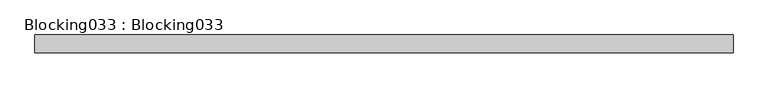
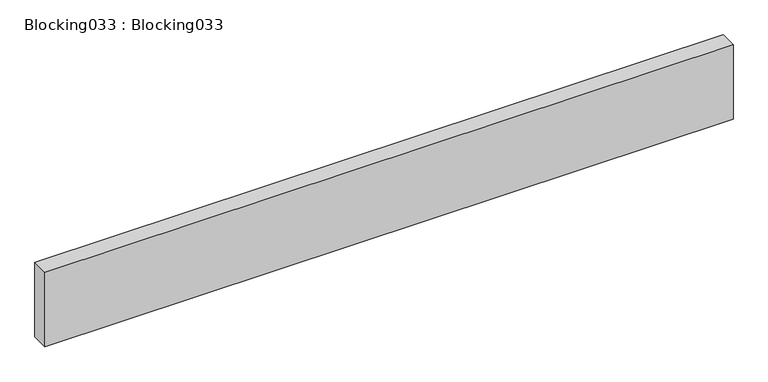
"""IFC4 building model written with IfcOpenShell, lengths in millimetres: proxy geometry, Blocking033 : Blocking033."""

from ifc_helpers import new_model, si_unit, frame, origin, place, context, project, spatial, polyline, outline, extrude, source, transform, mapped, element, save


def blocking033_blocking033_df2a4a9a(model_context):
    return source(origin(), model_context, "Body", "SweptSolid", [
        extrude(outline(polyline([(3694.2883192, 9592.4838724), (3694.2883192, 9643.2838724), (5694.2883192, 9643.2838724), (5694.2883192, 9592.4838724), (3694.2883192, 9592.4838724)])), frame((0.0, 0.0, 39528.496), z_axis=(0.0, 0.0, 1.0), x_axis=(1.0, 0.0, 0.0)), (0.0, 0.0, 1.0), 228.6),
    ])


if __name__ == "__main__":
    model = new_model("IFC4")
    model_context = context("Model", 3, world=origin())
    ifc_project = project(units=[si_unit("LENGTHUNIT", "METRE", prefix="MILLI")], contexts=[model_context])
    site = spatial("IfcSite", under=ifc_project)
    building = spatial("IfcBuilding", under=site)
    placement = place(None, origin())
    blocking033_blocking033_shape = blocking033_blocking033_df2a4a9a(model_context)
    element("IfcBuildingElementProxy", 1, Name="Blocking033 : Blocking033", ObjectType="Blocking033 : Blocking033", at=placement, inside=building, context=model_context, shape_type="MappedRepresentation", body=[
        mapped(blocking033_blocking033_shape, transform((0.0, 0.0, 0.0), x_axis=(1.0, 0.0, 0.0), y_axis=(0.0, 1.0, 0.0), z_axis=(0.0, 0.0, 1.0))),
    ])
    save(model, "model.ifc")

# Revit data of these elements
# Type "Blocking033 : Blocking033"
#   NameOverride = "Blocking033"
# Element 1 (IfcBuildingElementProxy, "Blocking033 : Blocking033")
#   Materials on its faces: "WOOD BLOCKING AS REQUIRED"
# Materials
#   "WOOD BLOCKING AS REQUIRED": class "Unassigned", colour RGB 166 124 85, transparency 0, Cost = 0
